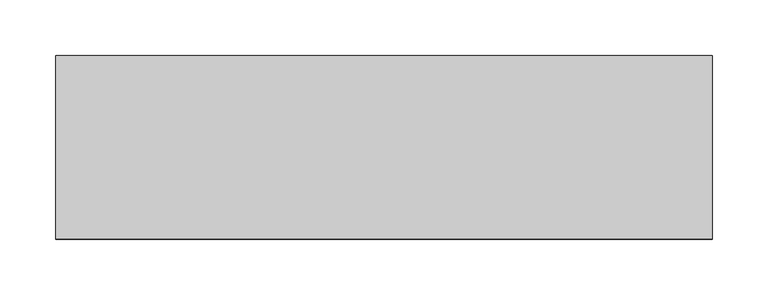
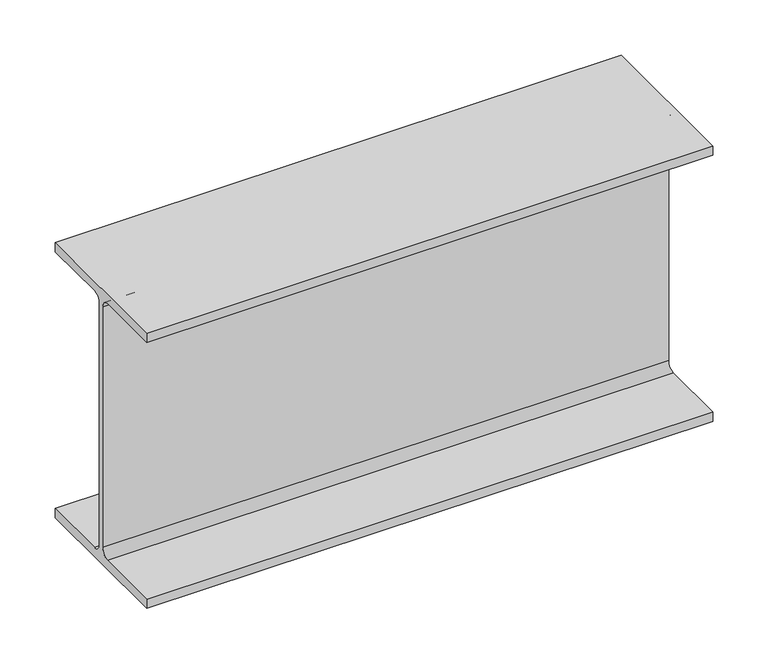
"""IFC4 building model written with IfcOpenShell, lengths in millimetres: beam geometry, Old_Steel Beam_H-KSD3502 : H_SB_ASB_H-300×150x6.5x9."""

from ifc_helpers import new_model, si_unit, point, frame, frame_2d, origin, place, context, project, spatial, polyline, circle_curve, trimmed, segment, composite_curve, outline, extrude, source, transform, mapped, element, save


def beam_aae560ba(model_context):
    return source(origin(), model_context, "Body", "SweptSolid", [
        extrude(outline(composite_curve([segment(polyline([(-82.5, -141.5), (-11.9, -141.5)]), True, "CONTINUOUS"), segment(trimmed(circle_curve(frame_2d((-11.9, -132.6)), 8.9), [point((-11.9, -141.5))], [point((-3.0, -132.6))], True, "CARTESIAN"), True, "CONTINUOUS"), segment(polyline([(-3.0, -132.6), (-3.0, 132.6)]), True, "CONTINUOUS"), segment(trimmed(circle_curve(frame_2d((-11.9, 132.6)), 8.9), [point((-3.0, 132.6))], [point((-11.9, 141.5))], True, "CARTESIAN"), True, "CONTINUOUS"), segment(polyline([(-11.9, 141.5), (-82.5, 141.5), (-82.5, 151.7), (82.5, 151.7), (82.5, 141.5), (11.9, 141.5)]), True, "CONTINUOUS"), segment(trimmed(circle_curve(frame_2d((11.9, 132.6)), 8.9), [point((11.9, 141.5))], [point((3.0, 132.6))], True, "CARTESIAN"), True, "CONTINUOUS"), segment(polyline([(3.0, 132.6), (3.0, -132.6)]), True, "CONTINUOUS"), segment(trimmed(circle_curve(frame_2d((11.9, -132.6)), 8.9), [point((3.0, -132.6))], [point((11.9, -141.5))], True, "CARTESIAN"), True, "CONTINUOUS"), segment(polyline([(11.9, -141.5), (82.5, -141.5), (82.5, -151.7), (-82.5, -151.7), (-82.5, -141.5)]), True, "CONTINUOUS")], self_intersect=False)), frame((-282.3, 0.0, 0.0), z_axis=(1.0, 0.0, 0.0), x_axis=(0.0, 1.0, 0.0)), (0.0, 0.0, 1.0), 589.6),
    ])


if __name__ == "__main__":
    model = new_model("IFC4")
    model_context = context("Model", 3, world=origin())
    ifc_project = project(units=[si_unit("LENGTHUNIT", "METRE", prefix="MILLI")], contexts=[model_context])
    site = spatial("IfcSite", under=ifc_project)
    building = spatial("IfcBuilding", under=site)
    placement = place(None, origin())
    beam_shape = beam_aae560ba(model_context)
    element("IfcBeam", 1, ObjectType="Old_Steel Beam_H-KSD3502 : H_SB_ASB_H-300×150x6.5x9", at=placement, inside=building, context=model_context, shape_type="MappedRepresentation", body=[
        mapped(beam_shape, transform((0.0, 0.0, 0.0), x_axis=(1.0, 0.0, 0.0), y_axis=(0.0, 1.0, 0.0), z_axis=(0.0, 0.0, 1.0))),
    ])
    save(model, "model.ifc")

# Revit data of these elements
# Type "Old_Steel Beam_H-KSD3502 : H_SB_ASB_H-300×150x6.5x9"
#   Width = 15.0 cm
#   Web Thickness = 0.65 cm
#   Web Fillet = 1.3 cm
#   Warping Constant = 107174.0 cm⁶
#   Torsional Moment of Inertia = 9.9539 cm⁴
#   Torsional Modulus = 1.0 cm³
#   Section Area = 46.78 cm²
#   Plastic Modulus weak axis = 105.0 cm³
#   Plastic Modulus strong axis = 542.0 cm³
#   Perimeter = 1.17 m²/m
#   Nominal Weight = 36.70 kgf/m
#   Moment of Inertia weak axis = 508.00 cm⁴
#   Moment of Inertia strong axis = 7210.00 cm⁴
#   Height = 30.0 cm
#   Flange Thickness = 0.9 cm
#   Elastic Modulus weak axis = 67.7 cm³
#   Elastic Modulus strong axis = 481.0 cm³
#   Centroid Vertical = 15.0 cm
#   Centroid Horizontal = 7.5 cm
#   Length [instance default] = 1.5240 m
#   Structural Material [instance default] = Steel, 45-345
#   Assembly Code = ""
# Element 1 (IfcBeam, "Old_Steel Beam_H-KSD3502 : H_SB_ASB_H-300×150x6.5x9")
#   Structural Material = none
# Materials
#   "Steel, 45-345": class "Metal", colour RGB 189 187 185, transparency 0, Description = "Steel 345 MPa", Cost = 0
